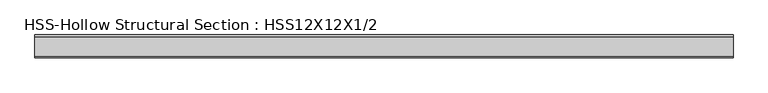
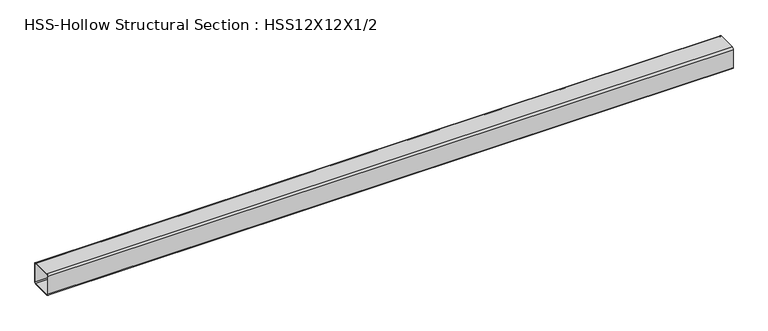
"""IFC4 building model written with IfcOpenShell, lengths in millimetres: beam geometry, HSS-Hollow Structural Section : HSS12X12X1/2."""

import ifcopenshell
import ifcopenshell.guid

model = None  # the IFC model being written
_history = None  # IfcOwnerHistory: only IFC2X3 demands one
_inside = {}  # id of a spatial element -> (the spatial element, [elements in it])
_under = {}  # id of a project, library or spatial element -> (it, [spatial elements below it])
_declared = {}  # id of a project -> (the project, [libraries it declares])
_typed = {}  # id of a type object -> (the type object, [elements of that type])
_made_of = {}  # id of a material, layer set ... -> (it, [elements and type objects made of it])


def new_model(schema):
    """Start an empty IFC model of exactly this schema.

    Asked for "IFC4X3", IfcOpenShell would pick the latest addendum, in which some entities
    have other attributes; the version numbers below select the first issue.
    IFC2X3 requires an IfcOwnerHistory on every rooted entity: one is made here for all.
    """
    global model, _history
    if schema == "IFC4X3":
        model = ifcopenshell.file(schema_version=(4, 3, 0, 0))
    else:
        model = ifcopenshell.file(schema=schema)
    _inside.clear()
    _under.clear()
    _declared.clear()
    _typed.clear()
    _made_of.clear()
    _history = None
    if model.schema == "IFC2X3":
        org = make("IfcOrganization", Name="unknown")
        user = make(
            "IfcPersonAndOrganization",
            ThePerson=make("IfcPerson", FamilyName="unknown"),
            TheOrganization=org,
        )
        app = make(
            "IfcApplication",
            ApplicationDeveloper=org,
            Version="unknown",
            ApplicationFullName="unknown",
            ApplicationIdentifier="unknown",
        )
        _history = make(
            "IfcOwnerHistory",
            OwningUser=user,
            OwningApplication=app,
            ChangeAction="ADDED",
            CreationDate=0,
        )
    return model


def make(cls, **values):
    """One entity of the class cls with the attributes given. An attribute that is None is left unset."""
    return model.create_entity(
        cls, **{name: value for name, value in values.items() if value is not None}
    )


def rooted(cls, **values):
    """An entity with a GlobalId (a new one), such as an element, a storey or a relation."""
    return make(cls, GlobalId=ifcopenshell.guid.new(), OwnerHistory=_history, **values)


def si_unit(unit_type, name, prefix=None):
    """IfcSIUnit, for example si_unit("LENGTHUNIT", "METRE", prefix="MILLI")."""
    return make("IfcSIUnit", UnitType=unit_type, Prefix=prefix, Name=name)


def assignment(units):
    """IfcUnitAssignment: the units of a project."""
    return None if units is None else make("IfcUnitAssignment", Units=units)


def point(xyz):
    """IfcCartesianPoint."""
    return None if xyz is None else make("IfcCartesianPoint", Coordinates=xyz)


def direction(xyz):
    """IfcDirection."""
    return None if xyz is None else make("IfcDirection", DirectionRatios=xyz)


def frame(location, z_axis=None, x_axis=None):
    """IfcAxis2Placement3D, a coordinate frame: its origin and axes. An axis left out is left unset."""
    return make(
        "IfcAxis2Placement3D",
        Location=point(location),
        Axis=direction(z_axis),
        RefDirection=direction(x_axis),
    )


def frame_2d(location, x_axis=None):
    """IfcAxis2Placement2D, a coordinate frame in the plane: its origin and x axis."""
    return make(
        "IfcAxis2Placement2D", Location=point(location), RefDirection=direction(x_axis)
    )


def origin():
    """The frame at (0, 0, 0) with its axes left unset."""
    return frame((0.0, 0.0, 0.0))


def place(relative_to, where):
    """IfcLocalPlacement: puts the frame where relative to a parent placement (None: the world)."""
    return make(
        "IfcLocalPlacement", PlacementRelTo=relative_to, RelativePlacement=where
    )


def context(
    kind, dimensions, precision=None, world=None, true_north=None, identifier=None
):
    """IfcGeometricRepresentationContext, for example the 3D "Model" context."""
    return make(
        "IfcGeometricRepresentationContext",
        ContextIdentifier=identifier,
        ContextType=kind,
        CoordinateSpaceDimension=dimensions,
        Precision=precision,
        WorldCoordinateSystem=world,
        TrueNorth=true_north,
    )


def project(units=None, contexts=None):
    """IfcProject with its units and contexts."""
    return rooted(
        "IfcProject",
        Name="project",
        RepresentationContexts=contexts,
        UnitsInContext=assignment(units),
    )


def spatial(cls, under=None, at=None, **own):
    """A site, building, storey or space (cls), placed at a placement, below another one or the project."""
    s = rooted(cls, ObjectPlacement=at, **own)
    if under is not None:
        _under.setdefault(under.id(), (under, []))[1].append(s)
    return s


def polyline(points):
    """IfcPolyline through the points."""
    return make("IfcPolyline", Points=[point(p) for p in points])


def circle_curve(where, radius):
    """IfcCircle in the frame where."""
    return make("IfcCircle", Position=where, Radius=radius)


def trimmed(basis, trim1, trim2, sense, master):
    """IfcTrimmedCurve: the piece of a basis curve between two trims."""
    return make(
        "IfcTrimmedCurve",
        BasisCurve=basis,
        Trim1=trim1,
        Trim2=trim2,
        SenseAgreement=sense,
        MasterRepresentation=master,
    )


def segment(curve, same_sense, transition):
    """IfcCompositeCurveSegment."""
    return make(
        "IfcCompositeCurveSegment",
        Transition=transition,
        SameSense=same_sense,
        ParentCurve=curve,
    )


def composite_curve(segments, self_intersect=None):
    """IfcCompositeCurve: segments joined end to end."""
    return make("IfcCompositeCurve", Segments=segments, SelfIntersect=self_intersect)


def outline(outer, holes=None, kind="AREA"):
    """IfcArbitraryClosedProfileDef: a profile drawn as a closed curve; with holes, ...WithVoids."""
    if holes is None:
        return make("IfcArbitraryClosedProfileDef", ProfileType=kind, OuterCurve=outer)
    return make(
        "IfcArbitraryProfileDefWithVoids",
        ProfileType=kind,
        OuterCurve=outer,
        InnerCurves=holes,
    )


def extrude(swept, where, along, depth):
    """IfcExtrudedAreaSolid: the profile swept, set in the frame where, extruded along a direction by depth."""
    return make(
        "IfcExtrudedAreaSolid",
        SweptArea=swept,
        Position=where,
        ExtrudedDirection=direction(along),
        Depth=depth,
    )


def shape(context_of_items, identifier, shape_type, items):
    """IfcShapeRepresentation: the items that make up one representation, for example the "Body"."""
    return make(
        "IfcShapeRepresentation",
        ContextOfItems=context_of_items,
        RepresentationIdentifier=identifier,
        RepresentationType=shape_type,
        Items=items,
    )


def source(mapping_origin, context_of_items, identifier, shape_type, items):
    """IfcRepresentationMap: a shape defined once, which mapped items show again and again."""
    return make(
        "IfcRepresentationMap",
        MappingOrigin=mapping_origin,
        MappedRepresentation=shape(context_of_items, identifier, shape_type, items),
    )


def transform(
    local_origin,
    x_axis=None,
    y_axis=None,
    z_axis=None,
    scale=None,
    scale2=None,
    scale3=None,
    uniform=True,
):
    """IfcCartesianTransformationOperator3D, or its non-uniform kind. x_axis, y_axis, z_axis: its Axis1, 2, 3."""
    if uniform:
        return make(
            "IfcCartesianTransformationOperator3D",
            Axis1=direction(x_axis),
            Axis2=direction(y_axis),
            LocalOrigin=point(local_origin),
            Scale=scale,
            Axis3=direction(z_axis),
        )
    return make(
        "IfcCartesianTransformationOperator3DnonUniform",
        Axis1=direction(x_axis),
        Axis2=direction(y_axis),
        LocalOrigin=point(local_origin),
        Scale=scale,
        Axis3=direction(z_axis),
        Scale2=scale2,
        Scale3=scale3,
    )


def mapped(mapping_source, mapping_target):
    """IfcMappedItem: shows the shape of a source again, moved by a transform."""
    return make(
        "IfcMappedItem", MappingSource=mapping_source, MappingTarget=mapping_target
    )


def made_of(thing, what):
    """Note that an element or type object is made of a material, layer set ...; save() writes the relation."""
    if what is not None:
        _made_of.setdefault(what.id(), (what, []))[1].append(thing)
    return thing


def element(
    cls,
    number,
    at=None,
    inside=None,
    cuts=None,
    type_object=None,
    material=None,
    context=None,
    identifier="Body",
    shape_type=None,
    held_by="IfcProductDefinitionShape",
    body=None,
    shapes=None,
    **own,
):
    """One element of the class cls, such as IfcWall. Its Tag is "e" and its number.

    at: its placement. inside: the storey or other place that contains it. cuts: it is an
    opening in that element (IfcRelVoidsElement). A single representation is given by context,
    identifier, shape_type and body (its items); several are given by shapes. held_by: the class
    of the entity that holds the representations. save() writes the other relations.
    """
    e = rooted(cls, Tag="e%d" % number, ObjectPlacement=at, **own)
    if body is not None:
        shapes = [shape(context, identifier, shape_type, body)]
    if shapes is not None:
        e.Representation = make(held_by, Representations=shapes)
    if inside is not None:
        _inside.setdefault(inside.id(), (inside, []))[1].append(e)
    if cuts is not None:
        rooted(
            "IfcRelVoidsElement", RelatingBuildingElement=cuts, RelatedOpeningElement=e
        )
    if type_object is not None:
        _typed.setdefault(type_object.id(), (type_object, []))[1].append(e)
    return made_of(e, material)


def aggregate(whole, parts):
    """IfcRelAggregates: a whole, such as a stair, and the parts it consists of."""
    return rooted("IfcRelAggregates", RelatingObject=whole, RelatedObjects=parts)


def save(model, path):
    """Write the relations noted so far, then the file.

    IfcRelAggregates (storeys below a building ...), IfcRelContainedInSpatialStructure (elements
    in a storey), IfcRelDefinesByType, IfcRelAssociatesMaterial and IfcRelDeclares: one each for
    every whole, place, type object, material and project.
    """
    for whole, parts in _under.values():
        aggregate(whole, parts)
    for where, things in _inside.values():
        rooted(
            "IfcRelContainedInSpatialStructure",
            RelatedElements=things,
            RelatingStructure=where,
        )
    for kind, things in _typed.values():
        rooted("IfcRelDefinesByType", RelatedObjects=things, RelatingType=kind)
    for what, things in _made_of.values():
        rooted("IfcRelAssociatesMaterial", RelatedObjects=things, RelatingMaterial=what)
    for by, libraries in _declared.values():
        rooted("IfcRelDeclares", RelatingContext=by, RelatedDefinitions=libraries)
    model.write(path)


def hss_hollow_structural_section_hss12x12x1_2_070f9e11(model_context):
    return source(origin(), model_context, "Body", "SweptSolid", [
        extrude(outline(composite_curve([segment(polyline([(152.4, 128.778), (152.4, -128.778)]), True, "CONTINUOUS"), segment(trimmed(circle_curve(frame_2d((128.778, -128.778)), 23.622), [point((152.4, -128.778))], [point((128.778, -152.4))], False, "CARTESIAN"), True, "CONTINUOUS"), segment(polyline([(128.778, -152.4), (-128.778, -152.4)]), True, "CONTINUOUS"), segment(trimmed(circle_curve(frame_2d((-128.778, -128.778)), 23.622), [point((-128.778, -152.4))], [point((-152.4, -128.778))], False, "CARTESIAN"), True, "CONTINUOUS"), segment(polyline([(-152.4, -128.778), (-152.4, 128.778)]), True, "CONTINUOUS"), segment(trimmed(circle_curve(frame_2d((-128.778, 128.778)), 23.622), [point((-152.4, 128.778))], [point((-128.778, 152.4))], False, "CARTESIAN"), True, "CONTINUOUS"), segment(polyline([(-128.778, 152.4), (128.778, 152.4)]), True, "CONTINUOUS"), segment(trimmed(circle_curve(frame_2d((128.778, 128.778)), 23.622), [point((128.778, 152.4))], [point((152.4, 128.778))], False, "CARTESIAN"), True, "CONTINUOUS")], self_intersect=False), holes=[composite_curve([segment(trimmed(circle_curve(frame_2d((-128.778, 128.778)), 11.811), [point((-128.778, 140.589))], [point((-140.589, 128.778))], True, "CARTESIAN"), True, "CONTINUOUS"), segment(polyline([(-140.589, 128.778), (-140.589, -128.778)]), True, "CONTINUOUS"), segment(trimmed(circle_curve(frame_2d((-128.778, -128.778)), 11.811), [point((-140.589, -128.778))], [point((-128.778, -140.589))], True, "CARTESIAN"), True, "CONTINUOUS"), segment(polyline([(-128.778, -140.589), (128.778, -140.589)]), True, "CONTINUOUS"), segment(trimmed(circle_curve(frame_2d((128.778, -128.778)), 11.811), [point((128.778, -140.589))], [point((140.589, -128.778))], True, "CARTESIAN"), True, "CONTINUOUS"), segment(polyline([(140.589, -128.778), (140.589, 128.778)]), True, "CONTINUOUS"), segment(trimmed(circle_curve(frame_2d((128.778, 128.778)), 11.811), [point((140.589, 128.778))], [point((128.778, 140.589))], True, "CARTESIAN"), True, "CONTINUOUS"), segment(polyline([(128.778, 140.589), (-128.778, 140.589)]), True, "CONTINUOUS")], self_intersect=False)]), frame((-4705.4245597, 0.0, 0.0), z_axis=(1.0, 0.0, 0.0), x_axis=(0.0, 1.0, 0.0)), (0.0, 0.0, 1.0), 9256.6663051),
    ])


if __name__ == "__main__":
    model = new_model("IFC4")
    model_context = context("Model", 3, world=origin())
    ifc_project = project(units=[si_unit("LENGTHUNIT", "METRE", prefix="MILLI")], contexts=[model_context])
    site = spatial("IfcSite", under=ifc_project)
    building = spatial("IfcBuilding", under=site)
    placement = place(None, origin())
    hss_hollow_structural_section_hss12x12x1_2_shape = hss_hollow_structural_section_hss12x12x1_2_070f9e11(model_context)
    element("IfcBeam", 1, ObjectType="HSS-Hollow Structural Section : HSS12X12X1/2", at=placement, inside=building, context=model_context, shape_type="MappedRepresentation", body=[
        mapped(hss_hollow_structural_section_hss12x12x1_2_shape, transform((0.0, 0.0, 0.0), x_axis=(1.0, 0.0, 0.0), y_axis=(0.0, 1.0, 0.0), z_axis=(0.0, 0.0, 1.0))),
    ])
    save(model, "model.ifc")

# Revit data of these elements
# Type "HSS-Hollow Structural Section : HSS12X12X1/2"
#   Assembly Code = "B10"
#   Shape = "Square"
#   W = 75.9
#   Ht = 304.8 mm
#   Length [instance default] = 1524 mm
#   b = 304.8 mm
#   kr = 23.622 mm
#   t = 11.811 mm
#   A = 0.0134838 m²
#   Structural Material [instance default] = Steel ASTM A500, Grade B, Rectangular and Square
# Element 1 (IfcBeam, "HSS-Hollow Structural Section : HSS12X12X1/2")
#   Structural Material = Aluminum 7175 T73 0 Hot Formed
#   Materials on its faces: "Aluminum 7175 T73 0 Hot Formed"
# Materials
#   "Steel ASTM A500, Grade B, Rectangular and Square": class "Metal", colour RGB 199 199 199, transparency 0, Description = "Carbon steel", Cost = 0
#   "Aluminum 7175 T73 0 Hot Formed": class "Metal", colour RGB 120 120 120, transparency 0, Description = "Physical material.", Cost = 0
